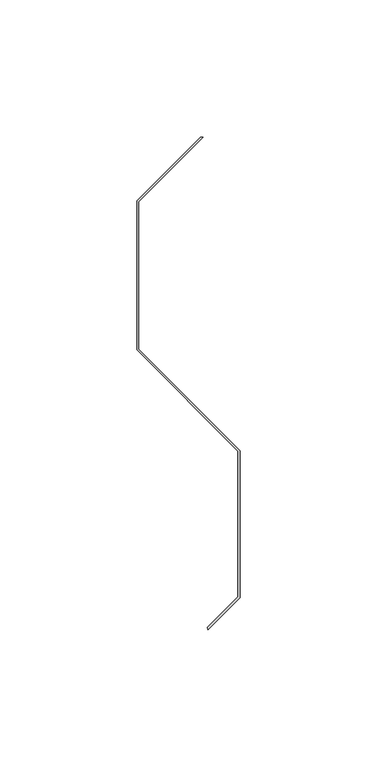
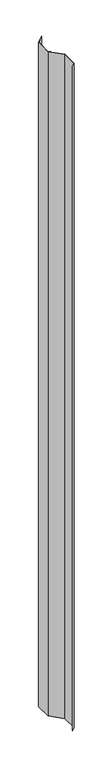
"""IFC4 building model written with IfcOpenShell, lengths in millimetres: proxy geometry, MBCI 7.2-V Panel11 : MBCI 7.2-V Panel-1."""

from ifc_helpers import new_model, si_unit, frame, origin, place, context, project, spatial, polyline, outline, extrude, source, transform, mapped, element, save


def generic_models_065db151(model_context):
    return source(origin(), model_context, "Body", "SweptSolid", [
        extrude(outline(polyline([(587365.2695864, -535322.081684), (587365.2695864, -535375.662984), (587353.5988637, -535387.3337068), (587353.54384, -535386.5468314), (587364.6742739, -535375.4163975), (587364.6742739, -535322.3282706), (587327.7791864, -535285.4331831), (587327.7791864, -535231.1525192), (587351.0153216, -535207.9163841), (587351.8572206, -535207.9163841), (587328.3744989, -535231.3991057), (587328.3744989, -535285.1865965), (587365.2695864, -535322.081684)])), frame((0.0, 0.0, 51.59375), z_axis=(0.0, 0.0, 1.0), x_axis=(1.0, 0.0, 0.0)), (0.0, 0.0, 1.0), 2386.80625),
    ])


if __name__ == "__main__":
    model = new_model("IFC4")
    model_context = context("Model", 3, world=origin())
    ifc_project = project(units=[si_unit("LENGTHUNIT", "METRE", prefix="MILLI")], contexts=[model_context])
    site = spatial("IfcSite", under=ifc_project)
    building = spatial("IfcBuilding", under=site)
    placement = place(None, origin())
    generic_models_shape = generic_models_065db151(model_context)
    element("IfcBuildingElementProxy", 1, Name="MBCI 7.2-V Panel11 : MBCI 7.2-V Panel-1", ObjectType="MBCI 7.2-V Panel11 : MBCI 7.2-V Panel-1", at=placement, inside=building, context=model_context, shape_type="MappedRepresentation", body=[
        mapped(generic_models_shape, transform((0.0, 0.0, 0.0), x_axis=(1.0, 0.0, 0.0), y_axis=(0.0, 1.0, 0.0), z_axis=(0.0, 0.0, 1.0))),
    ])
    save(model, "model.ifc")

# Revit data of these elements
# Element 1 (IfcBuildingElementProxy, "MBCI 7.2-V Panel11 : MBCI 7.2-V Panel-1")
#   Materials on its faces: "MTL PANEL"
# Materials
#   "MTL PANEL": class "Generic", colour RGB 239 242 240, transparency 0, Cost = 0
